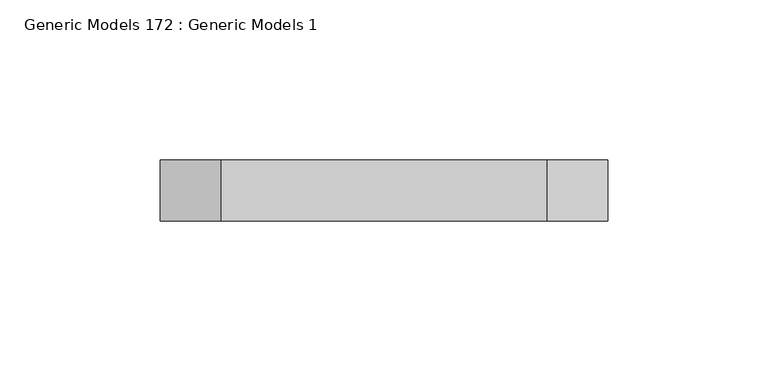
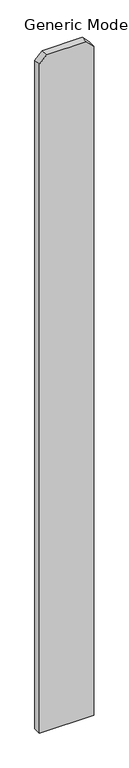
"""IFC4 building model written with IfcOpenShell, lengths in millimetres: proxy geometry, Generic Models 172 : Generic Models 1."""

from ifc_helpers import new_model, si_unit, frame, origin, place, context, project, spatial, polyline, outline, extrude, source, transform, mapped, element, save


def generic_models_172_generic_models_1_c27b7d85(model_context):
    return source(origin(), model_context, "Body", "SweptSolid", [
        extrude(outline(polyline([(76.2, -248591.3875), (1885.95, -248591.3875), (1905.0, -248610.4375), (1905.0, -248712.0375), (1885.95, -248731.0875), (76.2, -248731.0875), (76.2, -248591.3875)])), frame((0.0, 547.6875, 0.0), z_axis=(0.0, 1.0, 0.0), x_axis=(0.0, 0.0, 1.0)), (0.0, 0.0, 1.0), 19.05),
    ])


if __name__ == "__main__":
    model = new_model("IFC4")
    model_context = context("Model", 3, world=origin())
    ifc_project = project(units=[si_unit("LENGTHUNIT", "METRE", prefix="MILLI")], contexts=[model_context])
    site = spatial("IfcSite", under=ifc_project)
    building = spatial("IfcBuilding", under=site)
    placement = place(None, origin())
    generic_models_172_generic_models_1_shape = generic_models_172_generic_models_1_c27b7d85(model_context)
    element("IfcBuildingElementProxy", 1, Name="Generic Models 172 : Generic Models 1", ObjectType="Generic Models 172 : Generic Models 1", at=placement, inside=building, context=model_context, shape_type="MappedRepresentation", body=[
        mapped(generic_models_172_generic_models_1_shape, transform((0.0, 0.0, 0.0), x_axis=(1.0, 0.0, 0.0), y_axis=(0.0, 1.0, 0.0), z_axis=(0.0, 0.0, 1.0))),
    ])
    save(model, "model.ifc")

# Revit data of these elements
# Element 1 (IfcBuildingElementProxy, "Generic Models 172 : Generic Models 1")
#   Materials on its faces: "VERTICAL 1X6 CEDAR PLANKS W/ CLEAR WOOD SEALER"
# Materials
#   "VERTICAL 1X6 CEDAR PLANKS W/ CLEAR WOOD SEALER": class "Wood", colour RGB 234 198 147, transparency 0, Description = "Pinus Echinata", Cost = 0
